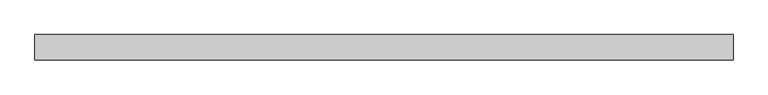
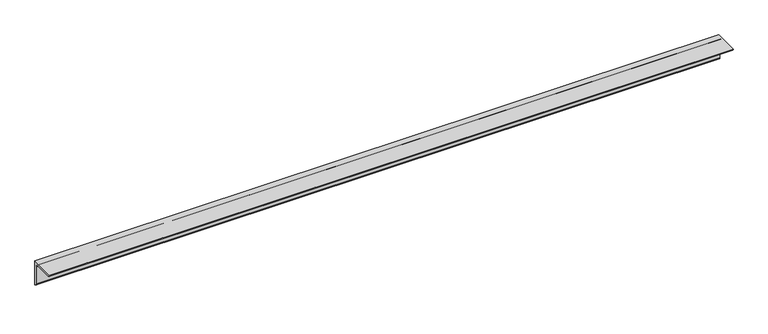
"""IFC4 building model written with IfcOpenShell, lengths in millimetres: beam geometry, 0912_Steel Framing_L-KSD3502 : H_SB_AR_S04_L-130x130x12_KBR1."""

from ifc_helpers import new_model, si_unit, point, frame, frame_2d, origin, place, context, project, spatial, polyline, circle_curve, trimmed, segment, composite_curve, outline, extrude, source, transform, mapped, element, save


def beam_14297e1c(model_context):
    return source(origin(), model_context, "Body", "SweptSolid", [
        extrude(outline(composite_curve([segment(polyline([(36.4, 36.4), (36.4, -93.6)]), True, "CONTINUOUS"), segment(trimmed(circle_curve(frame_2d((36.4, -81.6)), 12.0), [point((36.4, -93.6))], [point((24.4, -81.6))], False, "CARTESIAN"), True, "CONTINUOUS"), segment(polyline([(24.4, -81.6), (24.4, 12.4)]), True, "CONTINUOUS"), segment(trimmed(circle_curve(frame_2d((12.4, 12.4)), 12.0), [point((24.4, 12.4))], [point((12.4, 24.4))], True, "CARTESIAN"), True, "CONTINUOUS"), segment(polyline([(12.4, 24.4), (-81.6, 24.4)]), True, "CONTINUOUS"), segment(trimmed(circle_curve(frame_2d((-81.6, 36.4)), 12.0), [point((-81.6, 24.4))], [point((-93.6, 36.4))], False, "CARTESIAN"), True, "CONTINUOUS"), segment(polyline([(-93.6, 36.4), (36.4, 36.4)]), True, "CONTINUOUS")], self_intersect=False)), frame((-1819.863551, 0.0, 0.0), z_axis=(1.0, 0.0, 0.0), x_axis=(0.0, 1.0, 0.0)), (0.0, 0.0, 1.0), 3551.9244278),
    ])


if __name__ == "__main__":
    model = new_model("IFC4")
    model_context = context("Model", 3, world=origin())
    ifc_project = project(units=[si_unit("LENGTHUNIT", "METRE", prefix="MILLI")], contexts=[model_context])
    site = spatial("IfcSite", under=ifc_project)
    building = spatial("IfcBuilding", under=site)
    placement = place(None, origin())
    beam_shape = beam_14297e1c(model_context)
    element("IfcBeam", 1, ObjectType="0912_Steel Framing_L-KSD3502 : H_SB_AR_S04_L-130x130x12_KBR1", at=placement, inside=building, context=model_context, shape_type="MappedRepresentation", body=[
        mapped(beam_shape, transform((0.0, 0.0, 0.0), x_axis=(1.0, 0.0, 0.0), y_axis=(0.0, 1.0, 0.0), z_axis=(0.0, 0.0, 1.0))),
    ])
    save(model, "model.ifc")

# Revit data of these elements
# Type "0912_Steel Framing_L-KSD3502 : H_SB_AR_S04_L-130x130x12_KBR1"
#   k = 25 mm
#   Perimeter = 0.52 m²/m
#   Nominal Weight = 23.40 kgf/m
#   Length [instance default] = 1000 mm
#   b = 130 mm
#   d = 130 mm
#   t = 12 mm
#   x = 36.4 mm
#   y = 36.4 mm
#   A = 2976.00 m²
#   Structural Material [instance default] = Steel, 45-345
# Element 1 (IfcBeam, "0912_Steel Framing_L-KSD3502 : H_SB_AR_S04_L-130x130x12_KBR1")
#   Structural Material = Steel ASTM A36
#   Materials on its faces: "Steel ASTM A36"
# Materials
#   "Steel, 45-345": class "Metal", colour RGB 189 187 185, transparency 0, Description = "Steel 345 MPa", Cost = 0
#   "Steel ASTM A36": class "Metal", colour RGB 199 199 199, transparency 0, Description = "Structural steel, ASTM A36 Grade B, mill finish", Cost = 0
